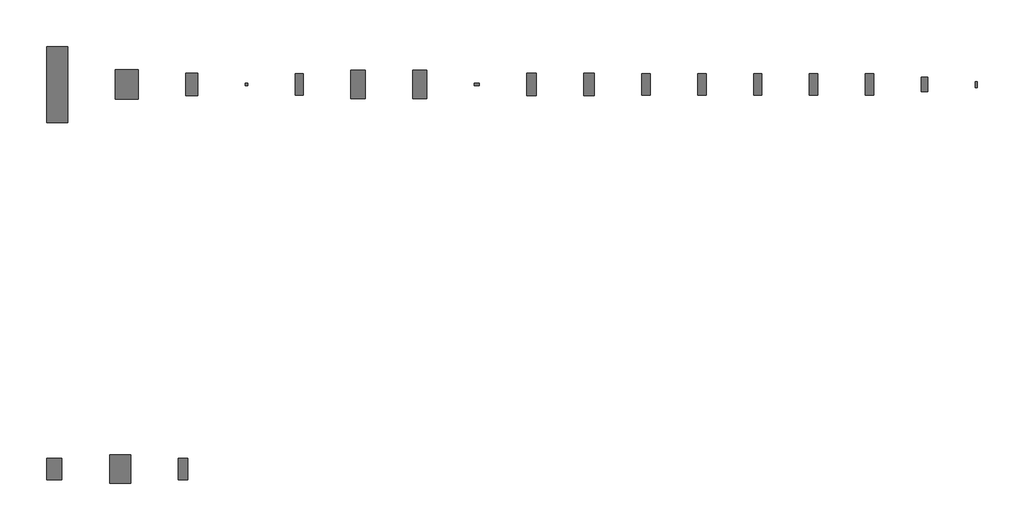
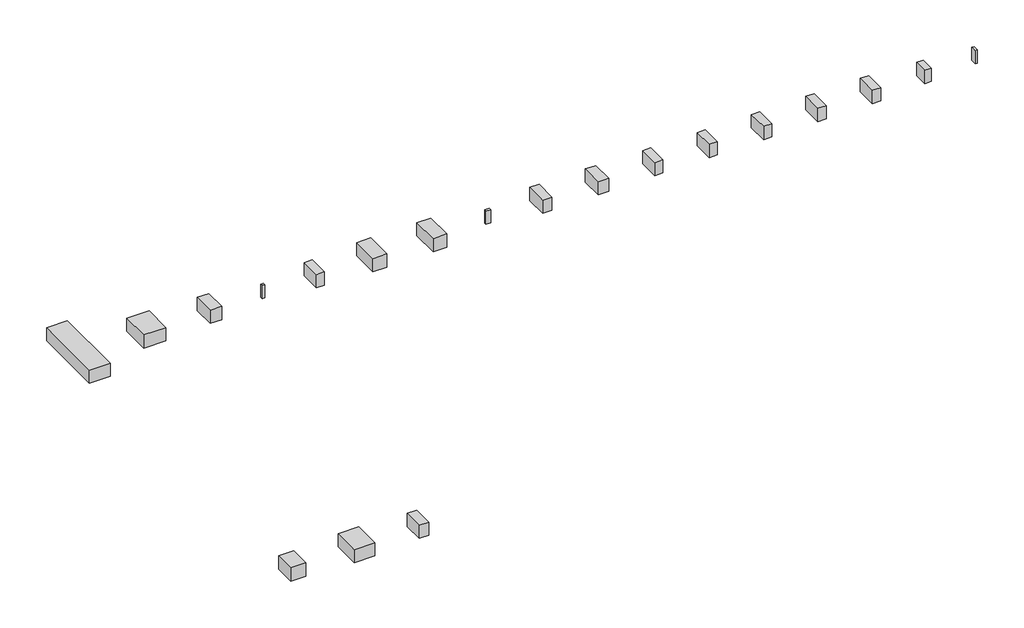
# One storey: 20 proxies.
"""IFC4 building model written with IfcOpenShell, lengths in millimetres."""

import ifcopenshell
import ifcopenshell.guid

model = None  # the IFC model being written
_history = None  # IfcOwnerHistory: only IFC2X3 demands one
_inside = {}  # id of a spatial element -> (the spatial element, [elements in it])
_under = {}  # id of a project, library or spatial element -> (it, [spatial elements below it])
_declared = {}  # id of a project -> (the project, [libraries it declares])
_typed = {}  # id of a type object -> (the type object, [elements of that type])
_made_of = {}  # id of a material, layer set ... -> (it, [elements and type objects made of it])


def new_model(schema):
    """Start an empty IFC model of exactly this schema.

    Asked for "IFC4X3", IfcOpenShell would pick the latest addendum, in which some entities
    have other attributes; the version numbers below select the first issue.
    IFC2X3 requires an IfcOwnerHistory on every rooted entity: one is made here for all.
    """
    global model, _history
    if schema == "IFC4X3":
        model = ifcopenshell.file(schema_version=(4, 3, 0, 0))
    else:
        model = ifcopenshell.file(schema=schema)
    _inside.clear()
    _under.clear()
    _declared.clear()
    _typed.clear()
    _made_of.clear()
    _history = None
    if model.schema == "IFC2X3":
        org = make("IfcOrganization", Name="unknown")
        user = make(
            "IfcPersonAndOrganization",
            ThePerson=make("IfcPerson", FamilyName="unknown"),
            TheOrganization=org,
        )
        app = make(
            "IfcApplication",
            ApplicationDeveloper=org,
            Version="unknown",
            ApplicationFullName="unknown",
            ApplicationIdentifier="unknown",
        )
        _history = make(
            "IfcOwnerHistory",
            OwningUser=user,
            OwningApplication=app,
            ChangeAction="ADDED",
            CreationDate=0,
        )
    return model


def make(cls, **values):
    """One entity of the class cls with the attributes given. An attribute that is None is left unset."""
    return model.create_entity(
        cls, **{name: value for name, value in values.items() if value is not None}
    )


def rooted(cls, **values):
    """An entity with a GlobalId (a new one), such as an element, a storey or a relation."""
    return make(cls, GlobalId=ifcopenshell.guid.new(), OwnerHistory=_history, **values)


def si_unit(unit_type, name, prefix=None):
    """IfcSIUnit, for example si_unit("LENGTHUNIT", "METRE", prefix="MILLI")."""
    return make("IfcSIUnit", UnitType=unit_type, Prefix=prefix, Name=name)


def assignment(units):
    """IfcUnitAssignment: the units of a project."""
    return None if units is None else make("IfcUnitAssignment", Units=units)


def point(xyz):
    """IfcCartesianPoint."""
    return None if xyz is None else make("IfcCartesianPoint", Coordinates=xyz)


def direction(xyz):
    """IfcDirection."""
    return None if xyz is None else make("IfcDirection", DirectionRatios=xyz)


def frame(location, z_axis=None, x_axis=None):
    """IfcAxis2Placement3D, a coordinate frame: its origin and axes. An axis left out is left unset."""
    return make(
        "IfcAxis2Placement3D",
        Location=point(location),
        Axis=direction(z_axis),
        RefDirection=direction(x_axis),
    )


def origin():
    """The frame at (0, 0, 0) with its axes left unset."""
    return frame((0.0, 0.0, 0.0))


def origin_with_axes():
    """The frame at (0, 0, 0) with the z axis (0, 0, 1) and the x axis (1, 0, 0) written out."""
    return frame((0.0, 0.0, 0.0), z_axis=(0.0, 0.0, 1.0), x_axis=(1.0, 0.0, 0.0))


def place(relative_to, where):
    """IfcLocalPlacement: puts the frame where relative to a parent placement (None: the world)."""
    return make(
        "IfcLocalPlacement", PlacementRelTo=relative_to, RelativePlacement=where
    )


def context(
    kind, dimensions, precision=None, world=None, true_north=None, identifier=None
):
    """IfcGeometricRepresentationContext, for example the 3D "Model" context."""
    return make(
        "IfcGeometricRepresentationContext",
        ContextIdentifier=identifier,
        ContextType=kind,
        CoordinateSpaceDimension=dimensions,
        Precision=precision,
        WorldCoordinateSystem=world,
        TrueNorth=true_north,
    )


def project(units=None, contexts=None):
    """IfcProject with its units and contexts."""
    return rooted(
        "IfcProject",
        Name="project",
        RepresentationContexts=contexts,
        UnitsInContext=assignment(units),
    )


def spatial(cls, under=None, at=None, **own):
    """A site, building, storey or space (cls), placed at a placement, below another one or the project."""
    s = rooted(cls, ObjectPlacement=at, **own)
    if under is not None:
        _under.setdefault(under.id(), (under, []))[1].append(s)
    return s


def polyline(points):
    """IfcPolyline through the points."""
    return make("IfcPolyline", Points=[point(p) for p in points])


def outline(outer, holes=None, kind="AREA"):
    """IfcArbitraryClosedProfileDef: a profile drawn as a closed curve; with holes, ...WithVoids."""
    if holes is None:
        return make("IfcArbitraryClosedProfileDef", ProfileType=kind, OuterCurve=outer)
    return make(
        "IfcArbitraryProfileDefWithVoids",
        ProfileType=kind,
        OuterCurve=outer,
        InnerCurves=holes,
    )


def extrude(swept, where, along, depth):
    """IfcExtrudedAreaSolid: the profile swept, set in the frame where, extruded along a direction by depth."""
    return make(
        "IfcExtrudedAreaSolid",
        SweptArea=swept,
        Position=where,
        ExtrudedDirection=direction(along),
        Depth=depth,
    )


def shape(context_of_items, identifier, shape_type, items):
    """IfcShapeRepresentation: the items that make up one representation, for example the "Body"."""
    return make(
        "IfcShapeRepresentation",
        ContextOfItems=context_of_items,
        RepresentationIdentifier=identifier,
        RepresentationType=shape_type,
        Items=items,
    )


def source(mapping_origin, context_of_items, identifier, shape_type, items):
    """IfcRepresentationMap: a shape defined once, which mapped items show again and again."""
    return make(
        "IfcRepresentationMap",
        MappingOrigin=mapping_origin,
        MappedRepresentation=shape(context_of_items, identifier, shape_type, items),
    )


def transform(
    local_origin,
    x_axis=None,
    y_axis=None,
    z_axis=None,
    scale=None,
    scale2=None,
    scale3=None,
    uniform=True,
):
    """IfcCartesianTransformationOperator3D, or its non-uniform kind. x_axis, y_axis, z_axis: its Axis1, 2, 3."""
    if uniform:
        return make(
            "IfcCartesianTransformationOperator3D",
            Axis1=direction(x_axis),
            Axis2=direction(y_axis),
            LocalOrigin=point(local_origin),
            Scale=scale,
            Axis3=direction(z_axis),
        )
    return make(
        "IfcCartesianTransformationOperator3DnonUniform",
        Axis1=direction(x_axis),
        Axis2=direction(y_axis),
        LocalOrigin=point(local_origin),
        Scale=scale,
        Axis3=direction(z_axis),
        Scale2=scale2,
        Scale3=scale3,
    )


def mapped(mapping_source, mapping_target):
    """IfcMappedItem: shows the shape of a source again, moved by a transform."""
    return make(
        "IfcMappedItem", MappingSource=mapping_source, MappingTarget=mapping_target
    )


def made_of(thing, what):
    """Note that an element or type object is made of a material, layer set ...; save() writes the relation."""
    if what is not None:
        _made_of.setdefault(what.id(), (what, []))[1].append(thing)
    return thing


def element(
    cls,
    number,
    at=None,
    inside=None,
    cuts=None,
    type_object=None,
    material=None,
    context=None,
    identifier="Body",
    shape_type=None,
    held_by="IfcProductDefinitionShape",
    body=None,
    shapes=None,
    **own,
):
    """One element of the class cls, such as IfcWall. Its Tag is "e" and its number.

    at: its placement. inside: the storey or other place that contains it. cuts: it is an
    opening in that element (IfcRelVoidsElement). A single representation is given by context,
    identifier, shape_type and body (its items); several are given by shapes. held_by: the class
    of the entity that holds the representations. save() writes the other relations.
    """
    e = rooted(cls, Tag="e%d" % number, ObjectPlacement=at, **own)
    if body is not None:
        shapes = [shape(context, identifier, shape_type, body)]
    if shapes is not None:
        e.Representation = make(held_by, Representations=shapes)
    if inside is not None:
        _inside.setdefault(inside.id(), (inside, []))[1].append(e)
    if cuts is not None:
        rooted(
            "IfcRelVoidsElement", RelatingBuildingElement=cuts, RelatedOpeningElement=e
        )
    if type_object is not None:
        _typed.setdefault(type_object.id(), (type_object, []))[1].append(e)
    return made_of(e, material)


def aggregate(whole, parts):
    """IfcRelAggregates: a whole, such as a stair, and the parts it consists of."""
    return rooted("IfcRelAggregates", RelatingObject=whole, RelatedObjects=parts)


def save(model, path):
    """Write the relations noted so far, then the file.

    IfcRelAggregates (storeys below a building ...), IfcRelContainedInSpatialStructure (elements
    in a storey), IfcRelDefinesByType, IfcRelAssociatesMaterial and IfcRelDeclares: one each for
    every whole, place, type object, material and project.
    """
    for whole, parts in _under.values():
        aggregate(whole, parts)
    for where, things in _inside.values():
        rooted(
            "IfcRelContainedInSpatialStructure",
            RelatedElements=things,
            RelatingStructure=where,
        )
    for kind, things in _typed.values():
        rooted("IfcRelDefinesByType", RelatedObjects=things, RelatingType=kind)
    for what, things in _made_of.values():
        rooted("IfcRelAssociatesMaterial", RelatedObjects=things, RelatingMaterial=what)
    for by, libraries in _declared.values():
        rooted("IfcRelDeclares", RelatingContext=by, RelatedDefinitions=libraries)
    model.write(path)


def generic_models_1d705098(model_context):
    return source(origin(), model_context, "Body", "SweptSolid", [
        extrude(outline(polyline([(3250.0, 4500.0), (3250.0, -4500.0), (-3250.0, -4500.0), (-3250.0, 4500.0), (3250.0, 4500.0)])), origin_with_axes(), (0.0, 0.0, 1.0), 6000.0),
    ])


def generic_models_399a6151(model_context):
    return source(origin(), model_context, "Body", "SweptSolid", [
        extrude(outline(polyline([(4500.0, 6000.0), (4500.0, -6000.0), (-4500.0, -6000.0), (-4500.0, 6000.0), (4500.0, 6000.0)])), origin_with_axes(), (0.0, 0.0, 1.0), 6000.0),
    ])


def generic_models_29bcd6f9(model_context):
    return source(origin(), model_context, "Body", "SweptSolid", [
        extrude(outline(polyline([(2000.0, 4500.0), (2000.0, -4500.0), (-2000.0, -4500.0), (-2000.0, 4500.0), (2000.0, 4500.0)])), origin_with_axes(), (0.0, 0.0, 1.0), 6000.0),
    ])


def generic_models_5634f436(model_context):
    return source(origin(), model_context, "Body", "SweptSolid", [
        extrude(outline(polyline([(1350.0, 3000.0), (1350.0, -3000.0), (-1350.0, -3000.0), (-1350.0, 3000.0), (1350.0, 3000.0)])), origin_with_axes(), (0.0, 0.0, 1.0), 6000.0),
    ])


def generic_models_71e2440f(model_context):
    return source(origin(), model_context, "Body", "SweptSolid", [
        extrude(outline(polyline([(500.0, 1250.0), (500.0, -1250.0), (-500.0, -1250.0), (-500.0, 1250.0), (500.0, 1250.0)])), origin_with_axes(), (0.0, 0.0, 1.0), 6000.0),
    ])


def generic_models_57c7875f(model_context):
    return source(origin(), model_context, "Body", "SweptSolid", [
        extrude(outline(polyline([(4500.0, 16000.0), (4500.0, -16000.0), (-4500.0, -16000.0), (-4500.0, 16000.0), (4500.0, 16000.0)])), origin_with_axes(), (0.0, 0.0, 1.0), 6000.0),
    ])


def generic_models_72d488a7(model_context):
    return source(origin(), model_context, "Body", "SweptSolid", [
        extrude(outline(polyline([(4800.0, 6250.0), (4800.0, -6250.0), (-4800.0, -6250.0), (-4800.0, 6250.0), (4800.0, 6250.0)])), origin_with_axes(), (0.0, 0.0, 1.0), 6000.0),
    ])


def generic_models_7902148a(model_context):
    return source(origin(), model_context, "Body", "SweptSolid", [
        extrude(outline(polyline([(2500.0, 4800.0), (2500.0, -4800.0), (-2500.0, -4800.0), (-2500.0, 4800.0), (2500.0, 4800.0)])), origin_with_axes(), (0.0, 0.0, 1.0), 6000.0),
    ])


def generic_models_ed4b717c(model_context):
    return source(origin(), model_context, "Body", "SweptSolid", [
        extrude(outline(polyline([(500.0, 500.0), (500.0, -500.0), (-500.0, -500.0), (-500.0, 500.0), (500.0, 500.0)])), origin_with_axes(), (0.0, 0.0, 1.0), 6000.0),
    ])


def generic_models_c01b8d6f(model_context):
    return source(origin(), model_context, "Body", "SweptSolid", [
        extrude(outline(polyline([(1750.0, 4500.0), (1750.0, -4500.0), (-1750.0, -4500.0), (-1750.0, 4500.0), (1750.0, 4500.0)])), origin_with_axes(), (0.0, 0.0, 1.0), 6000.0),
    ])


def generic_models_43059f4e(model_context):
    return source(origin(), model_context, "Body", "SweptSolid", [
        extrude(outline(polyline([(3000.0, 6000.0), (3000.0, -6000.0), (-3000.0, -6000.0), (-3000.0, 6000.0), (3000.0, 6000.0)])), origin_with_axes(), (0.0, 0.0, 1.0), 6000.0),
    ])


def generic_models_da00a96f(model_context):
    return source(origin(), model_context, "Body", "SweptSolid", [
        extrude(outline(polyline([(1000.0, 500.0), (1000.0, -500.0), (-1000.0, -500.0), (-1000.0, 500.0), (1000.0, 500.0)])), origin_with_axes(), (0.0, 0.0, 1.0), 6000.0),
    ])


def generic_models_3a820573(model_context):
    return source(origin(), model_context, "Body", "SweptSolid", [
        extrude(outline(polyline([(2000.0, 4750.0), (2000.0, -4750.0), (-2000.0, -4750.0), (-2000.0, 4750.0), (2000.0, 4750.0)])), origin_with_axes(), (0.0, 0.0, 1.0), 6000.0),
    ])


def generic_models_96097b63(model_context):
    return source(origin(), model_context, "Body", "SweptSolid", [
        extrude(outline(polyline([(2250.0, 4800.0), (2250.0, -4800.0), (-2250.0, -4800.0), (-2250.0, 4800.0), (2250.0, 4800.0)])), origin_with_axes(), (0.0, 0.0, 1.0), 6000.0),
    ])


model = new_model("IFC4")

# Units and contexts
model_context = context("Model", 3, world=origin())
ifc_project = project(units=[si_unit("LENGTHUNIT", "METRE", prefix="MILLI")], contexts=[model_context])

# Site, building, storey
site = spatial("IfcSite", under=ifc_project)
building = spatial("IfcBuilding", under=site)
storey = spatial("IfcBuildingStorey", under=building, Name="T.O.C_-1,300", Elevation=-1300.0)

# Proxies
placement = place(None, origin())
generic_models_shape = generic_models_1d705098(model_context)
element("IfcBuildingElementProxy", 1, Name="Space Planning Box_hec : Space Planning Box_hec", ObjectType="Space Planning Box_hec : Space Planning Box_hec", at=placement, inside=storey, context=model_context, shape_type="MappedRepresentation", body=[
    mapped(generic_models_shape, transform((3250.0, 6000.0, -300.0), x_axis=(1.0, 0.0, 0.0), y_axis=(0.0, 1.0, 0.0), z_axis=(0.0, 0.0, 1.0))),
])
generic_models_2_shape = generic_models_399a6151(model_context)
element("IfcBuildingElementProxy", 2, Name="Space Planning Box_hec : Space Planning Box_hec", ObjectType="Space Planning Box_hec : Space Planning Box_hec", at=placement, inside=storey, context=model_context, shape_type="MappedRepresentation", body=[
    mapped(generic_models_2_shape, transform((31000.0, 6000.0, -300.0), x_axis=(1.0, 0.0, 0.0), y_axis=(0.0, 1.0, 0.0), z_axis=(0.0, 0.0, 1.0))),
])
generic_models_3_shape = generic_models_29bcd6f9(model_context)
element("IfcBuildingElementProxy", 3, Name="Space Planning Box_hec : Space Planning Box_hec", ObjectType="Space Planning Box_hec : Space Planning Box_hec", at=placement, inside=storey, context=model_context, shape_type="MappedRepresentation", body=[
    mapped(generic_models_3_shape, transform((57500.0, 6000.0, -300.0), x_axis=(1.0, 0.0, 0.0), y_axis=(0.0, 1.0, 0.0), z_axis=(0.0, 0.0, 1.0))),
])
generic_models_4_shape = generic_models_5634f436(model_context)
element("IfcBuildingElementProxy", 4, Name="Space Planning Box_hec : Space Planning Box_hec", ObjectType="Space Planning Box_hec : Space Planning Box_hec", at=placement, inside=storey, context=model_context, shape_type="MappedRepresentation", body=[
    mapped(generic_models_4_shape, transform((369450.0, 168000.0, -1300.0), x_axis=(1.0, 0.0, 0.0), y_axis=(0.0, 1.0, 0.0), z_axis=(0.0, 0.0, 1.0))),
])
generic_models_5_shape = generic_models_71e2440f(model_context)
element("IfcBuildingElementProxy", 5, Name="Space Planning Box_hec : Space Planning Box_hec", ObjectType="Space Planning Box_hec : Space Planning Box_hec", at=placement, inside=storey, context=model_context, shape_type="MappedRepresentation", body=[
    mapped(generic_models_5_shape, transform((391300.0, 168000.0, -1300.0), x_axis=(1.0, 0.0, 0.0), y_axis=(0.0, 1.0, 0.0), z_axis=(0.0, 0.0, 1.0))),
])
generic_models_6_shape = generic_models_57c7875f(model_context)
element("IfcBuildingElementProxy", 6, Name="Space Planning Box_hec : Space Planning Box_hec", ObjectType="Space Planning Box_hec : Space Planning Box_hec", at=placement, inside=storey, context=model_context, shape_type="MappedRepresentation", body=[
    mapped(generic_models_6_shape, transform((4500.0, 168000.0, -1300.0), x_axis=(1.0, 0.0, 0.0), y_axis=(0.0, 1.0, 0.0), z_axis=(0.0, 0.0, 1.0))),
])
generic_models_7_shape = generic_models_72d488a7(model_context)
element("IfcBuildingElementProxy", 7, Name="Space Planning Box_hec : Space Planning Box_hec", ObjectType="Space Planning Box_hec : Space Planning Box_hec", at=placement, inside=storey, context=model_context, shape_type="MappedRepresentation", body=[
    mapped(generic_models_7_shape, transform((33800.0, 168000.0, -1300.0), x_axis=(1.0, 0.0, 0.0), y_axis=(0.0, 1.0, 0.0), z_axis=(0.0, 0.0, 1.0))),
])
generic_models_8_shape = generic_models_7902148a(model_context)
element("IfcBuildingElementProxy", 8, Name="Space Planning Box_hec : Space Planning Box_hec", ObjectType="Space Planning Box_hec : Space Planning Box_hec", at=placement, inside=storey, context=model_context, shape_type="MappedRepresentation", body=[
    mapped(generic_models_8_shape, transform((61100.0, 168000.0, -1300.0), x_axis=(1.0, 0.0, 0.0), y_axis=(0.0, 1.0, 0.0), z_axis=(0.0, 0.0, 1.0))),
])
generic_models_9_shape = generic_models_ed4b717c(model_context)
element("IfcBuildingElementProxy", 9, Name="Space Planning Box_hec : Space Planning Box_hec", ObjectType="Space Planning Box_hec : Space Planning Box_hec", at=placement, inside=storey, context=model_context, shape_type="MappedRepresentation", body=[
    mapped(generic_models_9_shape, transform((84100.0, 168000.0, -1300.0), x_axis=(1.0, 0.0, 0.0), y_axis=(0.0, 1.0, 0.0), z_axis=(0.0, 0.0, 1.0))),
])
generic_models_10_shape = generic_models_c01b8d6f(model_context)
element("IfcBuildingElementProxy", 10, Name="Space Planning Box_hec : Space Planning Box_hec", ObjectType="Space Planning Box_hec : Space Planning Box_hec", at=placement, inside=storey, context=model_context, shape_type="MappedRepresentation", body=[
    mapped(generic_models_10_shape, transform((106350.0, 168000.0, -1300.0), x_axis=(1.0, 0.0, 0.0), y_axis=(0.0, 1.0, 0.0), z_axis=(0.0, 0.0, 1.0))),
])
element("IfcBuildingElementProxy", 11, Name="Space Planning Box_hec : Space Planning Box_hec", ObjectType="Space Planning Box_hec : Space Planning Box_hec", at=placement, inside=storey, context=model_context, shape_type="MappedRepresentation", body=[
    mapped(generic_models_10_shape, transform((252350.0, 168000.0, -1300.0), x_axis=(1.0, 0.0, 0.0), y_axis=(0.0, 1.0, 0.0), z_axis=(0.0, 0.0, 1.0))),
])
element("IfcBuildingElementProxy", 12, Name="Space Planning Box_hec : Space Planning Box_hec", ObjectType="Space Planning Box_hec : Space Planning Box_hec", at=placement, inside=storey, context=model_context, shape_type="MappedRepresentation", body=[
    mapped(generic_models_10_shape, transform((275850.0, 168000.0, -1300.0), x_axis=(1.0, 0.0, 0.0), y_axis=(0.0, 1.0, 0.0), z_axis=(0.0, 0.0, 1.0))),
])
element("IfcBuildingElementProxy", 13, Name="Space Planning Box_hec : Space Planning Box_hec", ObjectType="Space Planning Box_hec : Space Planning Box_hec", at=placement, inside=storey, context=model_context, shape_type="MappedRepresentation", body=[
    mapped(generic_models_10_shape, transform((299350.0, 168000.0, -1300.0), x_axis=(1.0, 0.0, 0.0), y_axis=(0.0, 1.0, 0.0), z_axis=(0.0, 0.0, 1.0))),
])
element("IfcBuildingElementProxy", 14, Name="Space Planning Box_hec : Space Planning Box_hec", ObjectType="Space Planning Box_hec : Space Planning Box_hec", at=placement, inside=storey, context=model_context, shape_type="MappedRepresentation", body=[
    mapped(generic_models_10_shape, transform((322850.0, 168000.0, -1300.0), x_axis=(1.0, 0.0, 0.0), y_axis=(0.0, 1.0, 0.0), z_axis=(0.0, 0.0, 1.0))),
])
element("IfcBuildingElementProxy", 15, Name="Space Planning Box_hec : Space Planning Box_hec", ObjectType="Space Planning Box_hec : Space Planning Box_hec", at=placement, inside=storey, context=model_context, shape_type="MappedRepresentation", body=[
    mapped(generic_models_10_shape, transform((346350.0, 168000.0, -1300.0), x_axis=(1.0, 0.0, 0.0), y_axis=(0.0, 1.0, 0.0), z_axis=(0.0, 0.0, 1.0))),
])
generic_models_11_shape = generic_models_43059f4e(model_context)
element("IfcBuildingElementProxy", 16, Name="Space Planning Box_hec : Space Planning Box_hec", ObjectType="Space Planning Box_hec : Space Planning Box_hec", at=placement, inside=storey, context=model_context, shape_type="MappedRepresentation", body=[
    mapped(generic_models_11_shape, transform((131100.0, 168000.0, -1300.0), x_axis=(1.0, 0.0, 0.0), y_axis=(0.0, 1.0, 0.0), z_axis=(0.0, 0.0, 1.0))),
])
element("IfcBuildingElementProxy", 17, Name="Space Planning Box_hec : Space Planning Box_hec", ObjectType="Space Planning Box_hec : Space Planning Box_hec", at=placement, inside=storey, context=model_context, shape_type="MappedRepresentation", body=[
    mapped(generic_models_11_shape, transform((157100.0, 168000.0, -1300.0), x_axis=(1.0, 0.0, 0.0), y_axis=(0.0, 1.0, 0.0), z_axis=(0.0, 0.0, 1.0))),
])
generic_models_12_shape = generic_models_da00a96f(model_context)
element("IfcBuildingElementProxy", 18, Name="Space Planning Box_hec : Space Planning Box_hec", ObjectType="Space Planning Box_hec : Space Planning Box_hec", at=placement, inside=storey, context=model_context, shape_type="MappedRepresentation", body=[
    mapped(generic_models_12_shape, transform((181100.0, 168000.0, -1300.0), x_axis=(1.0, 0.0, 0.0), y_axis=(0.0, 1.0, 0.0), z_axis=(0.0, 0.0, 1.0))),
])
generic_models_13_shape = generic_models_3a820573(model_context)
element("IfcBuildingElementProxy", 19, Name="Space Planning Box_hec : Space Planning Box_hec", ObjectType="Space Planning Box_hec : Space Planning Box_hec", at=placement, inside=storey, context=model_context, shape_type="MappedRepresentation", body=[
    mapped(generic_models_13_shape, transform((204100.0, 168000.0, -1300.0), x_axis=(1.0, 0.0, 0.0), y_axis=(0.0, 1.0, 0.0), z_axis=(0.0, 0.0, 1.0))),
])
generic_models_14_shape = generic_models_96097b63(model_context)
element("IfcBuildingElementProxy", 20, Name="Space Planning Box_hec : Space Planning Box_hec", ObjectType="Space Planning Box_hec : Space Planning Box_hec", at=placement, inside=storey, context=model_context, shape_type="MappedRepresentation", body=[
    mapped(generic_models_14_shape, transform((228350.0, 168000.0, -1300.0), x_axis=(1.0, 0.0, 0.0), y_axis=(0.0, 1.0, 0.0), z_axis=(0.0, 0.0, 1.0))),
])

save(model, "model.ifc")

# Revit data of these elements
# Project information
#   Building Name = "MAIN GATE SECURITY BUILDING"
#   Project Status = "Project Status"
#   Client Name = "현대엔지니어링"
#   Project Address = "서울시 종로구 율곡로 75(계동)"
#   Project Name = "Therma Visayas Energy Project"
#   Project Number = "-"
# Grids (mm)
#   "A": line (0, 24502.793) -> (0, 11308.625)
#   "B": line (5000, 24502.793) -> (5000, 11308.625)
#   "C": line (10000, 24502.793) -> (10000, 11308.625)
#   "1": line (-3860.098, 13499.521) -> (12441.468, 13499.521)
#   "2": line (-3860.098, 20999.521) -> (12441.468, 20999.521)
# Type "Space Planning Box_hec : Space Planning Box_hec"
#   Type Comments = "..."
#   Room Name [instance default] = "?"
#   Interior Finish [instance default] = ""
#   Exterior Finish [instance default] = ""
#   Department [instance default] = ""
#   Assembly Code = "..."
#   Width [instance default] = 1524 mm
#   Program Area [instance default] = 0.00 m²
#   Length [instance default] = 1524 mm
#   Height [instance default] = 1524 mm
#   Area [instance default] = 2.32258 m²
#   Fill Color [instance default] = Cyan
#   Default Elevation = 0
# Element 1 (IfcBuildingElementProxy, "Space Planning Box_hec : Space Planning Box_hec")
#   Room Name = "Switchgear Room"
#   Interior Finish = "IF1"
#   Exterior Finish = "EF1"
#   Department = "EL"
#   Width = 6500 mm
#   Program Area = 58.50 m²
#   Length = 9000 mm
#   Height = 6000 mm
#   Area = 58.50 m²
#   Fill Color = Cyan
#   Phase Created = New Construction
#   Materials on its faces: "Cyan"
# Element 2 (IfcBuildingElementProxy, "Space Planning Box_hec : Space Planning Box_hec")
#   Room Name = "Battery Room"
#   Interior Finish = "IF4"
#   Exterior Finish = "EF1"
#   Department = "EL"
#   Width = 9000 mm
#   Program Area = 108.00 m²
#   Length = 12000 mm
#   Height = 6000 mm
#   Area = 108.00 m²
#   Fill Color = Cyan
#   Phase Created = New Construction
#   Materials on its faces: "Cyan"
# Element 3 (IfcBuildingElementProxy, "Space Planning Box_hec : Space Planning Box_hec")
#   Room Name = "Stairway"
#   Interior Finish = "IF2"
#   Exterior Finish = "EF1"
#   Department = "AR"
#   Width = 4000 mm
#   Program Area = 36.00 m²
#   Length = 9000 mm
#   Height = 6000 mm
#   Area = 36.00 m²
#   Fill Color = Cyan
#   Phase Created = New Construction
#   Materials on its faces: "Cyan"
# Element 4 (IfcBuildingElementProxy, "Space Planning Box_hec : Space Planning Box_hec")
#   Room Name = "Duct Shaft"
#   Interior Finish = "NA"
#   Exterior Finish = "EF1"
#   Department = "HV"
#   Width = 2700 mm
#   Program Area = 16.20 m²
#   Length = 6000 mm
#   Height = 6000 mm
#   Area = 16.20 m²
#   Fill Color = Cyan
#   Phase Created = New Construction
#   Materials on its faces: "Cyan"
# Element 5 (IfcBuildingElementProxy, "Space Planning Box_hec : Space Planning Box_hec")
#   Room Name = "Pipe Shaft"
#   Interior Finish = "NA"
#   Exterior Finish = "EF1"
#   Department = "HV"
#   Width = 1000 mm
#   Program Area = 2.50 m²
#   Length = 2500 mm
#   Height = 6000 mm
#   Area = 2.50 m²
#   Fill Color = Cyan
#   Phase Created = New Construction
#   Materials on its faces: "Cyan"
# Element 6 (IfcBuildingElementProxy, "Space Planning Box_hec : Space Planning Box_hec")
#   Room Name = "Central Control Room"
#   Interior Finish = "IF3"
#   Exterior Finish = "EF1"
#   Department = "CI"
#   Width = 9000 mm
#   Program Area = 288.00 m²
#   Length = 32000 mm
#   Height = 6000 mm
#   Area = 288.00 m²
#   Fill Color = Cyan
#   Phase Created = New Construction
#   Materials on its faces: "Cyan"
# Element 7 (IfcBuildingElementProxy, "Space Planning Box_hec : Space Planning Box_hec")
#   Room Name = "Engineer Room"
#   Interior Finish = "IF3"
#   Exterior Finish = "EF1"
#   Department = "CI"
#   Width = 9600 mm
#   Program Area = 120.00 m²
#   Length = 12500 mm
#   Height = 6000 mm
#   Area = 120.00 m²
#   Fill Color = Cyan
#   Phase Created = New Construction
#   Materials on its faces: "Cyan"
# Element 8 (IfcBuildingElementProxy, "Space Planning Box_hec : Space Planning Box_hec")
#   Room Name = "Document Room"
#   Interior Finish = "IF2-1"
#   Exterior Finish = "EF1"
#   Department = "AR"
#   Width = 5000 mm
#   Program Area = 48.00 m²
#   Length = 9600 mm
#   Height = 6000 mm
#   Area = 48.00 m²
#   Fill Color = Cyan
#   Phase Created = New Construction
#   Materials on its faces: "Cyan"
# Element 9 (IfcBuildingElementProxy, "Space Planning Box_hec : Space Planning Box_hec")
#   Room Name = "Fire Gas Room"
#   Interior Finish = "IF1"
#   Exterior Finish = "EF1"
#   Department = "SF"
#   Width = 1000 mm
#   Program Area = 0.00 m²
#   Length = 1000 mm
#   Height = 6000 mm
#   Area = 1.00 m²
#   Fill Color = Cyan
#   Phase Created = New Construction
#   Materials on its faces: "Cyan"
# Element 10 (IfcBuildingElementProxy, "Space Planning Box_hec : Space Planning Box_hec")
#   Room Name = "Kitch & Lunch Room"
#   Interior Finish = "IF2-1"
#   Exterior Finish = "EF1"
#   Department = "AR"
#   Width = 3500 mm
#   Program Area = 31.50 m²
#   Length = 9000 mm
#   Height = 6000 mm
#   Area = 31.50 m²
#   Fill Color = Cyan
#   Phase Created = New Construction
#   Materials on its faces: "Cyan"
# Element 11 (IfcBuildingElementProxy, "Space Planning Box_hec : Space Planning Box_hec")
#   Room Name = "LOTO Office Room"
#   Interior Finish = "IF2-1"
#   Exterior Finish = "EF1"
#   Department = "AR"
#   Width = 3500 mm
#   Program Area = 31.50 m²
#   Length = 9000 mm
#   Height = 6000 mm
#   Area = 31.50 m²
#   Fill Color = Cyan
#   Phase Created = New Construction
#   Materials on its faces: "Cyan"
# Element 12 (IfcBuildingElementProxy, "Space Planning Box_hec : Space Planning Box_hec")
#   Room Name = "Shower Room (F)"
#   Interior Finish = "IF5"
#   Exterior Finish = "EF1"
#   Department = "AR"
#   Width = 3500 mm
#   Program Area = 31.50 m²
#   Length = 9000 mm
#   Height = 6000 mm
#   Area = 31.50 m²
#   Fill Color = Cyan
#   Phase Created = New Construction
#   Materials on its faces: "Cyan"
# Element 13 (IfcBuildingElementProxy, "Space Planning Box_hec : Space Planning Box_hec")
#   Room Name = "Locker Room (F)"
#   Interior Finish = "IF2-1"
#   Exterior Finish = "EF1"
#   Department = "AR"
#   Width = 3500 mm
#   Program Area = 31.50 m²
#   Length = 9000 mm
#   Height = 6000 mm
#   Area = 31.50 m²
#   Fill Color = Cyan
#   Phase Created = New Construction
#   Materials on its faces: "Cyan"
# Element 14 (IfcBuildingElementProxy, "Space Planning Box_hec : Space Planning Box_hec")
#   Room Name = "Shower Room (M)"
#   Interior Finish = "IF5"
#   Exterior Finish = "EF1"
#   Department = "AR"
#   Width = 3500 mm
#   Program Area = 31.50 m²
#   Length = 9000 mm
#   Height = 6000 mm
#   Area = 31.50 m²
#   Fill Color = Cyan
#   Phase Created = New Construction
#   Materials on its faces: "Cyan"
# Element 15 (IfcBuildingElementProxy, "Space Planning Box_hec : Space Planning Box_hec")
#   Room Name = "Locker Room (M)"
#   Interior Finish = "IF2-1"
#   Exterior Finish = "EF1"
#   Department = "AR"
#   Width = 3500 mm
#   Program Area = 31.50 m²
#   Length = 9000 mm
#   Height = 6000 mm
#   Area = 31.50 m²
#   Fill Color = Cyan
#   Phase Created = New Construction
#   Materials on its faces: "Cyan"
# Element 16 (IfcBuildingElementProxy, "Space Planning Box_hec : Space Planning Box_hec")
#   Room Name = "Toilet (M)"
#   Interior Finish = "IF5"
#   Exterior Finish = "EF1"
#   Department = "AR"
#   Width = 6000 mm
#   Program Area = 72.00 m²
#   Length = 12000 mm
#   Height = 6000 mm
#   Area = 72.00 m²
#   Fill Color = Cyan
#   Phase Created = New Construction
#   Materials on its faces: "Cyan"
# Element 17 (IfcBuildingElementProxy, "Space Planning Box_hec : Space Planning Box_hec")
#   Room Name = "Toilet (F)"
#   Interior Finish = "IF5"
#   Exterior Finish = "EF1"
#   Department = "AR"
#   Width = 6000 mm
#   Program Area = 72.00 m²
#   Length = 12000 mm
#   Height = 6000 mm
#   Area = 72.00 m²
#   Fill Color = Cyan
#   Phase Created = New Construction
#   Materials on its faces: "Cyan"
# Element 18 (IfcBuildingElementProxy, "Space Planning Box_hec : Space Planning Box_hec")
#   Room Name = "Corridor"
#   Interior Finish = "IF2-1"
#   Exterior Finish = "EF1"
#   Department = "AR"
#   Width = 2000 mm
#   Program Area = 0.00 m²
#   Length = 1000 mm
#   Height = 6000 mm
#   Area = 2.00 m²
#   Fill Color = Cyan
#   Phase Created = New Construction
#   Materials on its faces: "Cyan"
# Element 19 (IfcBuildingElementProxy, "Space Planning Box_hec : Space Planning Box_hec")
#   Room Name = "Stairway"
#   Interior Finish = "IF2"
#   Exterior Finish = "EF1"
#   Department = "AR"
#   Width = 4000 mm
#   Program Area = 38.00 m²
#   Length = 9500 mm
#   Height = 6000 mm
#   Area = 38.00 m²
#   Fill Color = Cyan
#   Phase Created = New Construction
#   Materials on its faces: "Cyan"
# Element 20 (IfcBuildingElementProxy, "Space Planning Box_hec : Space Planning Box_hec")
#   Room Name = "Shift Office Room"
#   Interior Finish = "IF2-1"
#   Exterior Finish = "EF1"
#   Department = "AR"
#   Width = 4500 mm
#   Program Area = 43.20 m²
#   Length = 9600 mm
#   Height = 6000 mm
#   Area = 43.20 m²
#   Fill Color = Cyan
#   Phase Created = New Construction
#   Materials on its faces: "Cyan"
# Materials
#   "Cyan": class "Generic", colour RGB 0 255 255, transparency 0.2, Cost = 0
